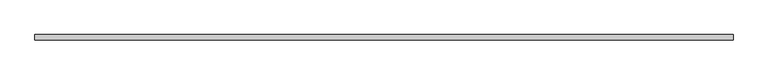
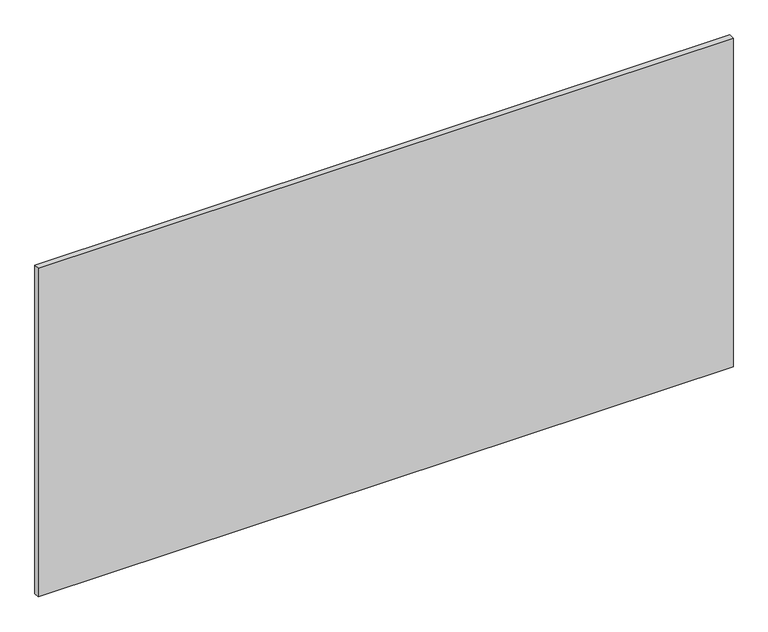
"""IFC4 building model written with IfcOpenShell, lengths in millimetres: proxy geometry, Inner panel:Inner panel:1:Inner panel:1 : Inner panel:Inner panel:300324:300043:Inner panel:1:Inner panel:1 : Inner panel:Inner panel:300324:300043 : Inner panel:Inner panel:1:Inner panel:1 : Inner panel:Inner panel:300324:300043:21 : Inner panel:Inner panel:1:Inner panel:1 : Inner panel:Inner panel:300324:300043:Inner panel:1:Inner panel:1 : Inner panel:Inner panel:300324:300043 : Inner panel:Inner panel:1:Inner panel:1 : Inner panel:Inner panel:300324:300043:300031."""

import ifcopenshell
import ifcopenshell.guid

model = None  # the IFC model being written
_history = None  # IfcOwnerHistory: only IFC2X3 demands one
_inside = {}  # id of a spatial element -> (the spatial element, [elements in it])
_under = {}  # id of a project, library or spatial element -> (it, [spatial elements below it])
_declared = {}  # id of a project -> (the project, [libraries it declares])
_typed = {}  # id of a type object -> (the type object, [elements of that type])
_made_of = {}  # id of a material, layer set ... -> (it, [elements and type objects made of it])


def new_model(schema):
    """Start an empty IFC model of exactly this schema.

    Asked for "IFC4X3", IfcOpenShell would pick the latest addendum, in which some entities
    have other attributes; the version numbers below select the first issue.
    IFC2X3 requires an IfcOwnerHistory on every rooted entity: one is made here for all.
    """
    global model, _history
    if schema == "IFC4X3":
        model = ifcopenshell.file(schema_version=(4, 3, 0, 0))
    else:
        model = ifcopenshell.file(schema=schema)
    _inside.clear()
    _under.clear()
    _declared.clear()
    _typed.clear()
    _made_of.clear()
    _history = None
    if model.schema == "IFC2X3":
        org = make("IfcOrganization", Name="unknown")
        user = make(
            "IfcPersonAndOrganization",
            ThePerson=make("IfcPerson", FamilyName="unknown"),
            TheOrganization=org,
        )
        app = make(
            "IfcApplication",
            ApplicationDeveloper=org,
            Version="unknown",
            ApplicationFullName="unknown",
            ApplicationIdentifier="unknown",
        )
        _history = make(
            "IfcOwnerHistory",
            OwningUser=user,
            OwningApplication=app,
            ChangeAction="ADDED",
            CreationDate=0,
        )
    return model


def make(cls, **values):
    """One entity of the class cls with the attributes given. An attribute that is None is left unset."""
    return model.create_entity(
        cls, **{name: value for name, value in values.items() if value is not None}
    )


def rooted(cls, **values):
    """An entity with a GlobalId (a new one), such as an element, a storey or a relation."""
    return make(cls, GlobalId=ifcopenshell.guid.new(), OwnerHistory=_history, **values)


def si_unit(unit_type, name, prefix=None):
    """IfcSIUnit, for example si_unit("LENGTHUNIT", "METRE", prefix="MILLI")."""
    return make("IfcSIUnit", UnitType=unit_type, Prefix=prefix, Name=name)


def assignment(units):
    """IfcUnitAssignment: the units of a project."""
    return None if units is None else make("IfcUnitAssignment", Units=units)


def point(xyz):
    """IfcCartesianPoint."""
    return None if xyz is None else make("IfcCartesianPoint", Coordinates=xyz)


def direction(xyz):
    """IfcDirection."""
    return None if xyz is None else make("IfcDirection", DirectionRatios=xyz)


def frame(location, z_axis=None, x_axis=None):
    """IfcAxis2Placement3D, a coordinate frame: its origin and axes. An axis left out is left unset."""
    return make(
        "IfcAxis2Placement3D",
        Location=point(location),
        Axis=direction(z_axis),
        RefDirection=direction(x_axis),
    )


def origin():
    """The frame at (0, 0, 0) with its axes left unset."""
    return frame((0.0, 0.0, 0.0))


def place(relative_to, where):
    """IfcLocalPlacement: puts the frame where relative to a parent placement (None: the world)."""
    return make(
        "IfcLocalPlacement", PlacementRelTo=relative_to, RelativePlacement=where
    )


def context(
    kind, dimensions, precision=None, world=None, true_north=None, identifier=None
):
    """IfcGeometricRepresentationContext, for example the 3D "Model" context."""
    return make(
        "IfcGeometricRepresentationContext",
        ContextIdentifier=identifier,
        ContextType=kind,
        CoordinateSpaceDimension=dimensions,
        Precision=precision,
        WorldCoordinateSystem=world,
        TrueNorth=true_north,
    )


def project(units=None, contexts=None):
    """IfcProject with its units and contexts."""
    return rooted(
        "IfcProject",
        Name="project",
        RepresentationContexts=contexts,
        UnitsInContext=assignment(units),
    )


def spatial(cls, under=None, at=None, **own):
    """A site, building, storey or space (cls), placed at a placement, below another one or the project."""
    s = rooted(cls, ObjectPlacement=at, **own)
    if under is not None:
        _under.setdefault(under.id(), (under, []))[1].append(s)
    return s


def polyline(points):
    """IfcPolyline through the points."""
    return make("IfcPolyline", Points=[point(p) for p in points])


def outline(outer, holes=None, kind="AREA"):
    """IfcArbitraryClosedProfileDef: a profile drawn as a closed curve; with holes, ...WithVoids."""
    if holes is None:
        return make("IfcArbitraryClosedProfileDef", ProfileType=kind, OuterCurve=outer)
    return make(
        "IfcArbitraryProfileDefWithVoids",
        ProfileType=kind,
        OuterCurve=outer,
        InnerCurves=holes,
    )


def extrude(swept, where, along, depth):
    """IfcExtrudedAreaSolid: the profile swept, set in the frame where, extruded along a direction by depth."""
    return make(
        "IfcExtrudedAreaSolid",
        SweptArea=swept,
        Position=where,
        ExtrudedDirection=direction(along),
        Depth=depth,
    )


def shape(context_of_items, identifier, shape_type, items):
    """IfcShapeRepresentation: the items that make up one representation, for example the "Body"."""
    return make(
        "IfcShapeRepresentation",
        ContextOfItems=context_of_items,
        RepresentationIdentifier=identifier,
        RepresentationType=shape_type,
        Items=items,
    )


def source(mapping_origin, context_of_items, identifier, shape_type, items):
    """IfcRepresentationMap: a shape defined once, which mapped items show again and again."""
    return make(
        "IfcRepresentationMap",
        MappingOrigin=mapping_origin,
        MappedRepresentation=shape(context_of_items, identifier, shape_type, items),
    )


def transform(
    local_origin,
    x_axis=None,
    y_axis=None,
    z_axis=None,
    scale=None,
    scale2=None,
    scale3=None,
    uniform=True,
):
    """IfcCartesianTransformationOperator3D, or its non-uniform kind. x_axis, y_axis, z_axis: its Axis1, 2, 3."""
    if uniform:
        return make(
            "IfcCartesianTransformationOperator3D",
            Axis1=direction(x_axis),
            Axis2=direction(y_axis),
            LocalOrigin=point(local_origin),
            Scale=scale,
            Axis3=direction(z_axis),
        )
    return make(
        "IfcCartesianTransformationOperator3DnonUniform",
        Axis1=direction(x_axis),
        Axis2=direction(y_axis),
        LocalOrigin=point(local_origin),
        Scale=scale,
        Axis3=direction(z_axis),
        Scale2=scale2,
        Scale3=scale3,
    )


def mapped(mapping_source, mapping_target):
    """IfcMappedItem: shows the shape of a source again, moved by a transform."""
    return make(
        "IfcMappedItem", MappingSource=mapping_source, MappingTarget=mapping_target
    )


def made_of(thing, what):
    """Note that an element or type object is made of a material, layer set ...; save() writes the relation."""
    if what is not None:
        _made_of.setdefault(what.id(), (what, []))[1].append(thing)
    return thing


def element(
    cls,
    number,
    at=None,
    inside=None,
    cuts=None,
    type_object=None,
    material=None,
    context=None,
    identifier="Body",
    shape_type=None,
    held_by="IfcProductDefinitionShape",
    body=None,
    shapes=None,
    **own,
):
    """One element of the class cls, such as IfcWall. Its Tag is "e" and its number.

    at: its placement. inside: the storey or other place that contains it. cuts: it is an
    opening in that element (IfcRelVoidsElement). A single representation is given by context,
    identifier, shape_type and body (its items); several are given by shapes. held_by: the class
    of the entity that holds the representations. save() writes the other relations.
    """
    e = rooted(cls, Tag="e%d" % number, ObjectPlacement=at, **own)
    if body is not None:
        shapes = [shape(context, identifier, shape_type, body)]
    if shapes is not None:
        e.Representation = make(held_by, Representations=shapes)
    if inside is not None:
        _inside.setdefault(inside.id(), (inside, []))[1].append(e)
    if cuts is not None:
        rooted(
            "IfcRelVoidsElement", RelatingBuildingElement=cuts, RelatedOpeningElement=e
        )
    if type_object is not None:
        _typed.setdefault(type_object.id(), (type_object, []))[1].append(e)
    return made_of(e, material)


def aggregate(whole, parts):
    """IfcRelAggregates: a whole, such as a stair, and the parts it consists of."""
    return rooted("IfcRelAggregates", RelatingObject=whole, RelatedObjects=parts)


def save(model, path):
    """Write the relations noted so far, then the file.

    IfcRelAggregates (storeys below a building ...), IfcRelContainedInSpatialStructure (elements
    in a storey), IfcRelDefinesByType, IfcRelAssociatesMaterial and IfcRelDeclares: one each for
    every whole, place, type object, material and project.
    """
    for whole, parts in _under.values():
        aggregate(whole, parts)
    for where, things in _inside.values():
        rooted(
            "IfcRelContainedInSpatialStructure",
            RelatedElements=things,
            RelatingStructure=where,
        )
    for kind, things in _typed.values():
        rooted("IfcRelDefinesByType", RelatedObjects=things, RelatingType=kind)
    for what, things in _made_of.values():
        rooted("IfcRelAssociatesMaterial", RelatedObjects=things, RelatingMaterial=what)
    for by, libraries in _declared.values():
        rooted("IfcRelDeclares", RelatingContext=by, RelatedDefinitions=libraries)
    model.write(path)


def generic_models_ae8239df(model_context):
    return source(origin(), model_context, "Body", "SweptSolid", [
        extrude(outline(polyline([(590067.7867239, -568186.6413841), (592506.1867239, -568186.6413841), (592506.1867239, -568205.6913841), (590067.7867239, -568205.6913841), (590067.7867239, -568186.6413841)])), frame((0.0, 0.0, 3721.1), z_axis=(0.0, 0.0, 1.0), x_axis=(1.0, 0.0, 0.0)), (0.0, 0.0, 1.0), 1219.2),
    ])


if __name__ == "__main__":
    model = new_model("IFC4")
    model_context = context("Model", 3, world=origin())
    ifc_project = project(units=[si_unit("LENGTHUNIT", "METRE", prefix="MILLI")], contexts=[model_context])
    site = spatial("IfcSite", under=ifc_project)
    building = spatial("IfcBuilding", under=site)
    placement = place(None, origin())
    generic_models_shape = generic_models_ae8239df(model_context)
    element("IfcBuildingElementProxy", 1, Name="Inner panel:Inner panel:1:Inner panel:1 : Inner panel:Inner panel:300324:300043:Inner panel:1:Inner panel:1 : Inner panel:Inner panel:300324:300043 : Inner panel:Inner panel:1:Inner panel:1 : Inner panel:Inner panel:300324:300043:21 : Inner panel:Inner panel:1:Inner panel:1 : Inner panel:Inner panel:300324:300043:Inner panel:1:Inner panel:1 : Inner panel:Inner panel:300324:300043 : Inner panel:Inner panel:1:Inner panel:1 : Inner panel:Inner panel:300324:300043:300031", ObjectType="Inner panel:Inner panel:1:Inner panel:1 : Inner panel:Inner panel:300324:300043:Inner panel:1:Inner panel:1 : Inner panel:Inner panel:300324:300043 : Inner panel:Inner panel:1:Inner panel:1 : Inner panel:Inner panel:300324:300043:21 : Inner panel:Inner panel:1:Inner panel:1 : Inner panel:Inner panel:300324:300043:Inner panel:1:Inner panel:1 : Inner panel:Inner panel:300324:300043 : Inner panel:Inner panel:1:Inner panel:1 : Inner panel:Inner panel:300324:300043:300031", at=placement, inside=building, context=model_context, shape_type="MappedRepresentation", body=[
        mapped(generic_models_shape, transform((0.0, 0.0, 0.0), x_axis=(1.0, 0.0, 0.0), y_axis=(0.0, 1.0, 0.0), z_axis=(0.0, 0.0, 1.0))),
    ])
    save(model, "model.ifc")

# Revit data of these elements
# Type "Inner panel:Inner panel:1:Inner panel:1 : Inner panel:Inner panel:300324:300043:Inner panel:1:Inner panel:1 : Inner panel:Inner panel:300324:300043 : Inner panel:Inner panel:1:Inner panel:1 : Inner panel:Inner panel:300324:300043:21 : Inner panel:Inner panel:1:Inner panel:1 : Inner panel:Inner panel:300324:300043:Inner panel:1:Inner panel:1 : Inner panel:Inner panel:300324:300043 : Inner panel:Inner panel:1:Inner panel:1 : Inner panel:Inner panel:300324:300043:300031"
#   NameOverride = "Inner panel:Inner panel:1:Inner panel:1 : Inner panel:Inner panel:300324:300043:Inner panel:1:Inner panel:1 : Inner panel:Inner panel:300324:300043 : Inner panel:Inner panel:1:Inner panel:1 : Inner panel:Inner panel:300324:300043:300031"
#   ObjectTypeOverride = "Inner panel:1:Inner panel:1 : Inner panel:Inner panel:300324:300043 : Inner panel:Inner panel:1:Inner panel:1 : Inner panel:Inner panel:300324:300043"
#   Reference = "Inner panel"
#   Tag = "300031"
# Element 1 (IfcBuildingElementProxy, "Inner panel:Inner panel:1:Inner panel:1 : Inner panel:Inner panel:300324:300043:Inner panel:1:Inner panel:1 : Inner panel:Inner panel:300324:300043 : Inner panel:Inner panel:1:Inner panel:1 : Inner panel:Inner panel:300324:300043:21 : Inner panel:Inner panel:1:Inner panel:1 : Inner panel:Inner panel:300324:300043:Inner panel:1:Inner panel:1 : Inner panel:Inner panel:300324:300043 : Inner panel:Inner panel:1:Inner panel:1 : Inner panel:Inner panel:300324:300043:300031")
#   Materials on its faces: "¾” (CLASS A) FIRE RETARDANT PLYWOOD ...OR… IF 1/4\" GYP. BD UNDER PLYWOOD, FLAME SPREAD TO BE CLASS C -  (FINISH: GRADE B - PREFINISHED STAINED/SEALED) - 1/4\" GAP BTWN PANELS (FASTENERS T.B.D.)"
# Materials
#   "¾” (CLASS A) FIRE RETARDANT PLYWOOD ...OR… IF 1/4\" GYP. BD UNDER PLYWOOD, FLAME SPREAD TO BE CLASS C -  (FINISH: GRADE B - PREFINISHED STAINED/SEALED) - 1/4\" GAP BTWN PANELS (FASTENERS T.B.D.)": class "Wood", colour RGB 149 120 74, transparency 0, Description = "Plywood, sheathing grade", Cost = 0
